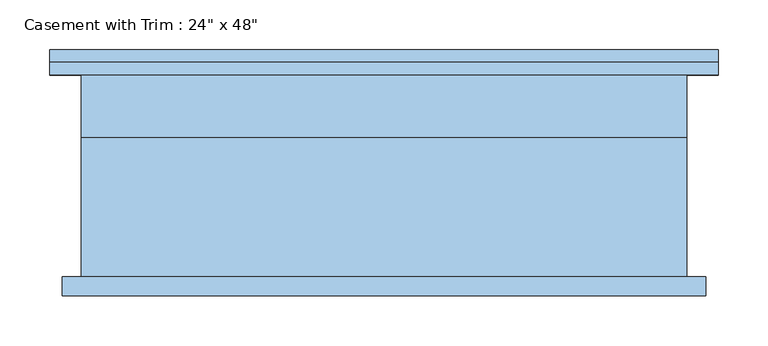
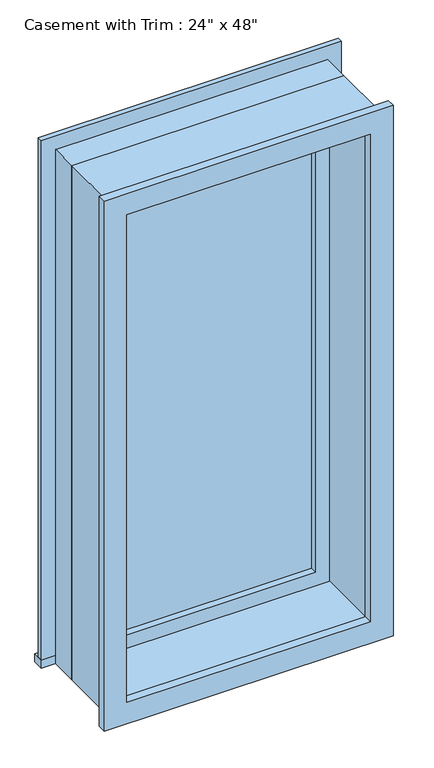
"""IFC4 building model written with IfcOpenShell, lengths in millimetres: window geometry."""

import ifcopenshell
import ifcopenshell.guid

model = None  # the IFC model being written
_history = None  # IfcOwnerHistory: only IFC2X3 demands one
_inside = {}  # id of a spatial element -> (the spatial element, [elements in it])
_under = {}  # id of a project, library or spatial element -> (it, [spatial elements below it])
_declared = {}  # id of a project -> (the project, [libraries it declares])
_typed = {}  # id of a type object -> (the type object, [elements of that type])
_made_of = {}  # id of a material, layer set ... -> (it, [elements and type objects made of it])


def new_model(schema):
    """Start an empty IFC model of exactly this schema.

    Asked for "IFC4X3", IfcOpenShell would pick the latest addendum, in which some entities
    have other attributes; the version numbers below select the first issue.
    IFC2X3 requires an IfcOwnerHistory on every rooted entity: one is made here for all.
    """
    global model, _history
    if schema == "IFC4X3":
        model = ifcopenshell.file(schema_version=(4, 3, 0, 0))
    else:
        model = ifcopenshell.file(schema=schema)
    _inside.clear()
    _under.clear()
    _declared.clear()
    _typed.clear()
    _made_of.clear()
    _history = None
    if model.schema == "IFC2X3":
        org = make("IfcOrganization", Name="unknown")
        user = make(
            "IfcPersonAndOrganization",
            ThePerson=make("IfcPerson", FamilyName="unknown"),
            TheOrganization=org,
        )
        app = make(
            "IfcApplication",
            ApplicationDeveloper=org,
            Version="unknown",
            ApplicationFullName="unknown",
            ApplicationIdentifier="unknown",
        )
        _history = make(
            "IfcOwnerHistory",
            OwningUser=user,
            OwningApplication=app,
            ChangeAction="ADDED",
            CreationDate=0,
        )
    return model


def make(cls, **values):
    """One entity of the class cls with the attributes given. An attribute that is None is left unset."""
    return model.create_entity(
        cls, **{name: value for name, value in values.items() if value is not None}
    )


def rooted(cls, **values):
    """An entity with a GlobalId (a new one), such as an element, a storey or a relation."""
    return make(cls, GlobalId=ifcopenshell.guid.new(), OwnerHistory=_history, **values)


def si_unit(unit_type, name, prefix=None):
    """IfcSIUnit, for example si_unit("LENGTHUNIT", "METRE", prefix="MILLI")."""
    return make("IfcSIUnit", UnitType=unit_type, Prefix=prefix, Name=name)


def assignment(units):
    """IfcUnitAssignment: the units of a project."""
    return None if units is None else make("IfcUnitAssignment", Units=units)


def point(xyz):
    """IfcCartesianPoint."""
    return None if xyz is None else make("IfcCartesianPoint", Coordinates=xyz)


def direction(xyz):
    """IfcDirection."""
    return None if xyz is None else make("IfcDirection", DirectionRatios=xyz)


def frame(location, z_axis=None, x_axis=None):
    """IfcAxis2Placement3D, a coordinate frame: its origin and axes. An axis left out is left unset."""
    return make(
        "IfcAxis2Placement3D",
        Location=point(location),
        Axis=direction(z_axis),
        RefDirection=direction(x_axis),
    )


def origin():
    """The frame at (0, 0, 0) with its axes left unset."""
    return frame((0.0, 0.0, 0.0))


def place(relative_to, where):
    """IfcLocalPlacement: puts the frame where relative to a parent placement (None: the world)."""
    return make(
        "IfcLocalPlacement", PlacementRelTo=relative_to, RelativePlacement=where
    )


def context(
    kind, dimensions, precision=None, world=None, true_north=None, identifier=None
):
    """IfcGeometricRepresentationContext, for example the 3D "Model" context."""
    return make(
        "IfcGeometricRepresentationContext",
        ContextIdentifier=identifier,
        ContextType=kind,
        CoordinateSpaceDimension=dimensions,
        Precision=precision,
        WorldCoordinateSystem=world,
        TrueNorth=true_north,
    )


def project(units=None, contexts=None):
    """IfcProject with its units and contexts."""
    return rooted(
        "IfcProject",
        Name="project",
        RepresentationContexts=contexts,
        UnitsInContext=assignment(units),
    )


def spatial(cls, under=None, at=None, **own):
    """A site, building, storey or space (cls), placed at a placement, below another one or the project."""
    s = rooted(cls, ObjectPlacement=at, **own)
    if under is not None:
        _under.setdefault(under.id(), (under, []))[1].append(s)
    return s


def polyline(points):
    """IfcPolyline through the points."""
    return make("IfcPolyline", Points=[point(p) for p in points])


def outline(outer, holes=None, kind="AREA"):
    """IfcArbitraryClosedProfileDef: a profile drawn as a closed curve; with holes, ...WithVoids."""
    if holes is None:
        return make("IfcArbitraryClosedProfileDef", ProfileType=kind, OuterCurve=outer)
    return make(
        "IfcArbitraryProfileDefWithVoids",
        ProfileType=kind,
        OuterCurve=outer,
        InnerCurves=holes,
    )


def extrude(swept, where, along, depth):
    """IfcExtrudedAreaSolid: the profile swept, set in the frame where, extruded along a direction by depth."""
    return make(
        "IfcExtrudedAreaSolid",
        SweptArea=swept,
        Position=where,
        ExtrudedDirection=direction(along),
        Depth=depth,
    )


def shape(context_of_items, identifier, shape_type, items):
    """IfcShapeRepresentation: the items that make up one representation, for example the "Body"."""
    return make(
        "IfcShapeRepresentation",
        ContextOfItems=context_of_items,
        RepresentationIdentifier=identifier,
        RepresentationType=shape_type,
        Items=items,
    )


def source(mapping_origin, context_of_items, identifier, shape_type, items):
    """IfcRepresentationMap: a shape defined once, which mapped items show again and again."""
    return make(
        "IfcRepresentationMap",
        MappingOrigin=mapping_origin,
        MappedRepresentation=shape(context_of_items, identifier, shape_type, items),
    )


def transform(
    local_origin,
    x_axis=None,
    y_axis=None,
    z_axis=None,
    scale=None,
    scale2=None,
    scale3=None,
    uniform=True,
):
    """IfcCartesianTransformationOperator3D, or its non-uniform kind. x_axis, y_axis, z_axis: its Axis1, 2, 3."""
    if uniform:
        return make(
            "IfcCartesianTransformationOperator3D",
            Axis1=direction(x_axis),
            Axis2=direction(y_axis),
            LocalOrigin=point(local_origin),
            Scale=scale,
            Axis3=direction(z_axis),
        )
    return make(
        "IfcCartesianTransformationOperator3DnonUniform",
        Axis1=direction(x_axis),
        Axis2=direction(y_axis),
        LocalOrigin=point(local_origin),
        Scale=scale,
        Axis3=direction(z_axis),
        Scale2=scale2,
        Scale3=scale3,
    )


def mapped(mapping_source, mapping_target):
    """IfcMappedItem: shows the shape of a source again, moved by a transform."""
    return make(
        "IfcMappedItem", MappingSource=mapping_source, MappingTarget=mapping_target
    )


def made_of(thing, what):
    """Note that an element or type object is made of a material, layer set ...; save() writes the relation."""
    if what is not None:
        _made_of.setdefault(what.id(), (what, []))[1].append(thing)
    return thing


def element(
    cls,
    number,
    at=None,
    inside=None,
    cuts=None,
    type_object=None,
    material=None,
    context=None,
    identifier="Body",
    shape_type=None,
    held_by="IfcProductDefinitionShape",
    body=None,
    shapes=None,
    **own,
):
    """One element of the class cls, such as IfcWall. Its Tag is "e" and its number.

    at: its placement. inside: the storey or other place that contains it. cuts: it is an
    opening in that element (IfcRelVoidsElement). A single representation is given by context,
    identifier, shape_type and body (its items); several are given by shapes. held_by: the class
    of the entity that holds the representations. save() writes the other relations.
    """
    e = rooted(cls, Tag="e%d" % number, ObjectPlacement=at, **own)
    if body is not None:
        shapes = [shape(context, identifier, shape_type, body)]
    if shapes is not None:
        e.Representation = make(held_by, Representations=shapes)
    if inside is not None:
        _inside.setdefault(inside.id(), (inside, []))[1].append(e)
    if cuts is not None:
        rooted(
            "IfcRelVoidsElement", RelatingBuildingElement=cuts, RelatedOpeningElement=e
        )
    if type_object is not None:
        _typed.setdefault(type_object.id(), (type_object, []))[1].append(e)
    return made_of(e, material)


def aggregate(whole, parts):
    """IfcRelAggregates: a whole, such as a stair, and the parts it consists of."""
    return rooted("IfcRelAggregates", RelatingObject=whole, RelatedObjects=parts)


def save(model, path):
    """Write the relations noted so far, then the file.

    IfcRelAggregates (storeys below a building ...), IfcRelContainedInSpatialStructure (elements
    in a storey), IfcRelDefinesByType, IfcRelAssociatesMaterial and IfcRelDeclares: one each for
    every whole, place, type object, material and project.
    """
    for whole, parts in _under.values():
        aggregate(whole, parts)
    for where, things in _inside.values():
        rooted(
            "IfcRelContainedInSpatialStructure",
            RelatedElements=things,
            RelatingStructure=where,
        )
    for kind, things in _typed.values():
        rooted("IfcRelDefinesByType", RelatedObjects=things, RelatingType=kind)
    for what, things in _made_of.values():
        rooted("IfcRelAssociatesMaterial", RelatedObjects=things, RelatingMaterial=what)
    for by, libraries in _declared.values():
        rooted("IfcRelDeclares", RelatingContext=by, RelatedDefinitions=libraries)
    model.write(path)


def window_21430ea7(model_context):
    return source(origin(), model_context, "Body", "SweptSolid", [
        extrude(outline(polyline([(-336.55, 127.0), (336.55, 127.0), (336.55, 101.6), (-336.55, 101.6), (-336.55, 127.0)])), frame((0.0, 0.0, 914.4), z_axis=(0.0, 0.0, 1.0), x_axis=(1.0, 0.0, 0.0)), (0.0, 0.0, 1.0), 19.05),
        extrude(outline(polyline([(2114.55, -285.75), (2114.55, 285.75), (933.45, 285.75), (933.45, 336.55), (2165.35, 336.55), (2165.35, -336.55), (933.45, -336.55), (933.45, -285.75), (2114.55, -285.75)])), frame((0.0, 101.6, 0.0), z_axis=(0.0, 1.0, 0.0), x_axis=(0.0, 0.0, 1.0)), (0.0, 0.0, 1.0), 12.7),
        extrude(outline(polyline([(2152.65, 323.85), (2152.65, -323.85), (895.35, -323.85), (895.35, 323.85), (2152.65, 323.85)]), holes=[polyline([(2101.85, 273.05), (946.15, 273.05), (946.15, -273.05), (2101.85, -273.05), (2101.85, 273.05)])]), frame((0.0, -120.65, 0.0), z_axis=(0.0, 1.0, 0.0), x_axis=(0.0, 0.0, 1.0)), (0.0, 0.0, 1.0), 19.05),
        extrude(outline(polyline([(241.3, 53.975), (-241.3, 53.975), (-241.3, 66.675), (241.3, 66.675), (241.3, 53.975)])), frame((0.0, 0.0, 977.9), z_axis=(0.0, 0.0, 1.0), x_axis=(1.0, 0.0, 0.0)), (0.0, 0.0, 1.0), 1092.2),
        extrude(outline(polyline([(2114.55, -285.75), (933.45, -285.75), (933.45, 285.75), (2114.55, 285.75), (2114.55, -285.75)]), holes=[polyline([(2070.1, -241.3), (2070.1, 241.3), (977.9, 241.3), (977.9, -241.3), (2070.1, -241.3)])]), frame((0.0, 38.1, 0.0), z_axis=(0.0, 1.0, 0.0), x_axis=(0.0, 0.0, 1.0)), (0.0, 0.0, 1.0), 44.45),
        extrude(outline(polyline([(2133.6, -304.8), (914.4, -304.8), (914.4, 304.8), (2133.6, 304.8), (2133.6, -304.8)]), holes=[polyline([(2101.85, -273.05), (2101.85, 273.05), (946.15, 273.05), (946.15, -273.05), (2101.85, -273.05)])]), frame((0.0, -101.6, 0.0), z_axis=(0.0, 1.0, 0.0), x_axis=(0.0, 0.0, 1.0)), (0.0, 0.0, 1.0), 139.7),
        extrude(outline(polyline([(2133.6, 304.8), (2133.6, -304.8), (914.4, -304.8), (914.4, 304.8), (2133.6, 304.8)]), holes=[polyline([(2114.55, 285.75), (933.45, 285.75), (933.45, -285.75), (2114.55, -285.75), (2114.55, 285.75)])]), frame((0.0, 38.1, 0.0), z_axis=(0.0, 1.0, 0.0), x_axis=(0.0, 0.0, 1.0)), (0.0, 0.0, 1.0), 63.5),
    ])


if __name__ == "__main__":
    model = new_model("IFC4")
    model_context = context("Model", 3, world=origin())
    ifc_project = project(units=[si_unit("LENGTHUNIT", "METRE", prefix="MILLI")], contexts=[model_context])
    site = spatial("IfcSite", under=ifc_project)
    building = spatial("IfcBuilding", under=site)
    placement = place(None, origin())
    window_shape = window_21430ea7(model_context)
    element("IfcWindow", 1, ObjectType="Casement with Trim : 24\" x 48\"", at=placement, inside=building, context=model_context, shape_type="MappedRepresentation", body=[
        mapped(window_shape, transform((0.0, 0.0, 0.0), x_axis=(1.0, 0.0, 0.0), y_axis=(0.0, 1.0, 0.0), z_axis=(0.0, 0.0, 1.0))),
    ])
    save(model, "model.ifc")

# Revit data of these elements
# Project information
#   Project Issue Date = "Issue Date"
#   Project Status = "Project Status"
#   Client Name = "Owner"
#   Project Address = "Enter address here"
#   Project Name = "Project Name"
#   Project Number = "Project Number"
#   SR Document GUID = "d5a3456e-cf0d-421d-b81f-9384e84516ce"
# Type "Casement with Trim : 24\" x 48\""
#   Type Mark = "39"
#   Assembly Code = "B2020100"
#   Height = 1219.20 mm
#   Default Sill Height = 914.40 mm
#   Trim Projection - Ext. = 12.70 mm
#   Trim Projection - Int. = 19.05 mm
#   Trim Width - Exterior = 50.80 mm
#   Trim Width - Interior = 50.80 mm
#   Width = 609.60 mm
#   Window Inset = 19.05 mm
#   Glass Pane Material = Glass
#   Sash Material = Sash
#   Trim Exterior Material = Trim
#   Trim Interior Material = Trim
#   Wall Closure = (empty or 0)
# Element 1 (IfcWindow, "Casement with Trim : 24\" x 48\"")
#   Materials on its faces: "Sash", "Trim", "Glass"
# Materials
#   "Glass": class "Glass", colour RGB 0 128 192, transparency 0.75
#   "Sash": class "Wood", colour RGB 224 178 126, transparency 0
#   "Trim": class "Wood", colour RGB 224 178 126, transparency 0
